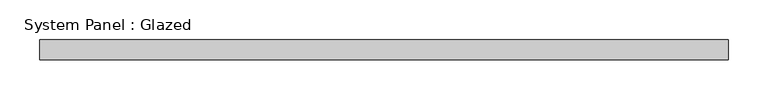
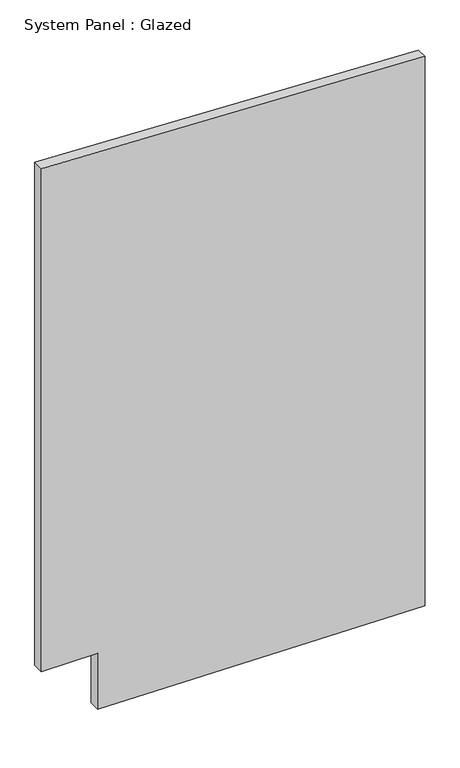
"""IFC4 building model written with IfcOpenShell, lengths in millimetres: plate geometry, System Panel : Glazed."""

from ifc_helpers import new_model, si_unit, frame, origin, place, context, project, spatial, polyline, outline, extrude, source, transform, mapped, element, save


def system_panel_glazed_776f7ef8(model_context):
    return source(origin(), model_context, "Body", "SweptSolid", [
        extrude(outline(polyline([(12.5542209, -307.3323712), (0.0, 434.3323712), (1313.8161075, 434.3323712), (1350.0104717, -434.3323712), (146.5743087, -434.3323712), (146.5743087, -307.3323712), (12.5542209, -307.3323712)])), frame((0.0, -12.7, 0.0), z_axis=(0.0, 1.0, 0.0), x_axis=(0.0, 0.0, 1.0)), (0.0, 0.0, 1.0), 25.4),
    ])


if __name__ == "__main__":
    model = new_model("IFC4")
    model_context = context("Model", 3, world=origin())
    ifc_project = project(units=[si_unit("LENGTHUNIT", "METRE", prefix="MILLI")], contexts=[model_context])
    site = spatial("IfcSite", under=ifc_project)
    building = spatial("IfcBuilding", under=site)
    placement = place(None, origin())
    system_panel_glazed_shape = system_panel_glazed_776f7ef8(model_context)
    element("IfcPlate", 1, ObjectType="System Panel : Glazed", at=placement, inside=building, context=model_context, shape_type="MappedRepresentation", body=[
        mapped(system_panel_glazed_shape, transform((0.0, 0.0, 0.0), x_axis=(1.0, 0.0, 0.0), y_axis=(0.0, 1.0, 0.0), z_axis=(0.0, 0.0, 1.0))),
    ])
    save(model, "model.ifc")

# Revit data of these elements
# Element 1 (IfcPlate, "System Panel : Glazed")
#   Materials on its faces: "BUTT GLAZED STOREFRONT WITH VERTICAL MULLION"
# Materials
#   "BUTT GLAZED STOREFRONT WITH VERTICAL MULLION": class "Glass", colour RGB 236 240 239, transparency 0.39, Description = "Soda Lime Glass", Cost = 0
